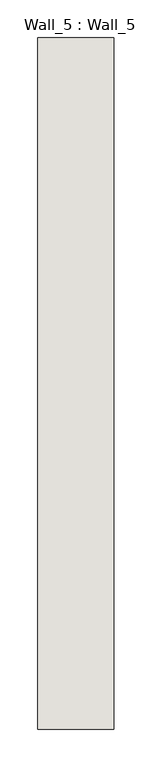
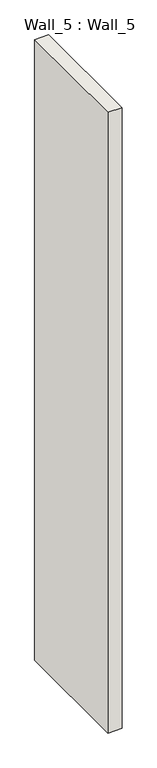
"""IFC4 building model written with IfcOpenShell, lengths in millimetres: wall geometry, Wall_5 : Wall_5."""

from ifc_helpers import new_model, si_unit, origin, origin_with_axes, place, context, project, spatial, polyline, outline, extrude, source, transform, mapped, element, save


def wall_5_wall_5_558b8a57(model_context):
    return source(origin(), model_context, "Body", "SweptSolid", [
        extrude(outline(polyline([(100.0, 16990.0), (100.0, 16080.0), (0.0, 16080.0), (0.0, 16990.0), (100.0, 16990.0)])), origin_with_axes(), (0.0, 0.0, 1.0), 4700.0),
    ])


if __name__ == "__main__":
    model = new_model("IFC4")
    model_context = context("Model", 3, world=origin())
    ifc_project = project(units=[si_unit("LENGTHUNIT", "METRE", prefix="MILLI")], contexts=[model_context])
    site = spatial("IfcSite", under=ifc_project)
    building = spatial("IfcBuilding", under=site)
    placement = place(None, origin())
    wall_5_wall_5_shape = wall_5_wall_5_558b8a57(model_context)
    element("IfcWall", 1, ObjectType="Wall_5 : Wall_5", at=placement, inside=building, context=model_context, shape_type="MappedRepresentation", body=[
        mapped(wall_5_wall_5_shape, transform((0.0, 0.0, 0.0), x_axis=(1.0, 0.0, 0.0), y_axis=(0.0, 1.0, 0.0), z_axis=(0.0, 0.0, 1.0))),
    ])
    save(model, "model.ifc")

# Revit data of these elements
# Type "Wall_5 : Wall_5"
#   NameOverride = "Wall_5"
# Element 1 (IfcWall, "Wall_5 : Wall_5")
#   Materials on its faces: "IfcSurfaceStyle #33"
# Materials
#   "IfcSurfaceStyle #33": class "Unassigned", colour RGB 214 214 214, transparency 0
